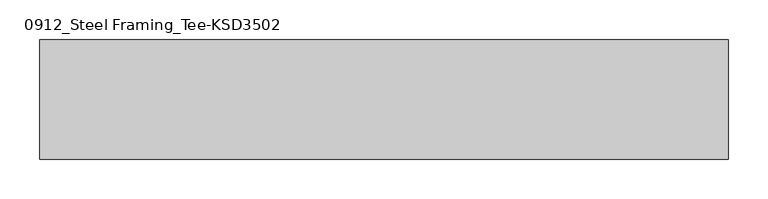
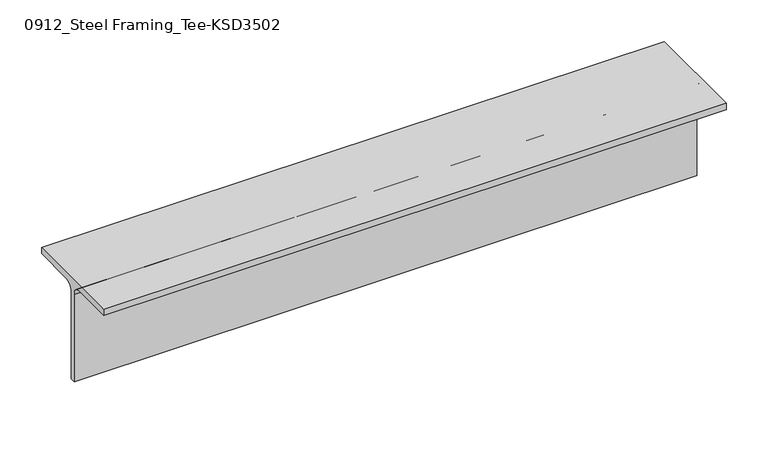
"""IFC4 building model written with IfcOpenShell, lengths in millimetres: member geometry, 0912_Steel Framing_Tee-KSD3502 : H_SB_ASB_CT-150x150x6.5x9."""

from ifc_helpers import new_model, si_unit, point, frame, frame_2d, origin, place, context, project, spatial, polyline, circle_curve, trimmed, segment, composite_curve, outline, extrude, source, transform, mapped, element, save


def member_0912_steel_framing_tee_ksd3502_ed30f98e(model_context):
    return source(origin(), model_context, "Body", "SweptSolid", [
        extrude(outline(composite_curve([segment(polyline([(-75.0, 75.0), (75.0, 75.0), (75.0, 66.0), (16.25, 66.0)]), True, "CONTINUOUS"), segment(trimmed(circle_curve(frame_2d((16.25, 53.0)), 13.0), [point((16.25, 66.0))], [point((3.25, 53.0))], True, "CARTESIAN"), True, "CONTINUOUS"), segment(polyline([(3.25, 53.0), (3.25, -75.0), (-3.25, -75.0), (-3.25, 53.0)]), True, "CONTINUOUS"), segment(trimmed(circle_curve(frame_2d((-16.25, 53.0)), 13.0), [point((-3.25, 53.0))], [point((-16.25, 66.0))], True, "CARTESIAN"), True, "CONTINUOUS"), segment(polyline([(-16.25, 66.0), (-75.0, 66.0), (-75.0, 75.0)]), True, "CONTINUOUS")], self_intersect=False)), frame((-365.9, 0.0, 0.0), z_axis=(1.0, 0.0, 0.0), x_axis=(0.0, 1.0, 0.0)), (0.0, 0.0, 1.0), 865.9),
    ])


if __name__ == "__main__":
    model = new_model("IFC4")
    model_context = context("Model", 3, world=origin())
    ifc_project = project(units=[si_unit("LENGTHUNIT", "METRE", prefix="MILLI")], contexts=[model_context])
    site = spatial("IfcSite", under=ifc_project)
    building = spatial("IfcBuilding", under=site)
    placement = place(None, origin())
    member_0912_steel_framing_tee_ksd3502_shape = member_0912_steel_framing_tee_ksd3502_ed30f98e(model_context)
    element("IfcMember", 1, ObjectType="0912_Steel Framing_Tee-KSD3502 : H_SB_ASB_CT-150x150x6.5x9", at=placement, inside=building, context=model_context, shape_type="MappedRepresentation", body=[
        mapped(member_0912_steel_framing_tee_ksd3502_shape, transform((0.0, 0.0, 0.0), x_axis=(1.0, 0.0, 0.0), y_axis=(0.0, 1.0, 0.0), z_axis=(0.0, 0.0, 1.0))),
    ])
    save(model, "model.ifc")

# Revit data of these elements
# Type "0912_Steel Framing_Tee-KSD3502 : H_SB_ASB_CT-150x150x6.5x9"
#   H_WM Code_1 = "S01AA003-00001 | Main Steel Structure Fabrication Work | Shelter/Building | Light Steel - Standard (30KG/M>Weight) | Material: (   )"
#   H_WM Code_2 = "S03AA029-00001 | Main Steel Structure Erection Work | Shelter/Building | Light Steel (30KG/M>Weight) | Material: (   )"
#   H_WM Code_3 = "S01AA010-00001 | Main Steel Structure Fabrication Work | Shelter/Building | Steel Painting/Coating | for Non-Fireproofed Steel Surface, Surface Preparation, Primer, Second & Final Coat | Material: (   )"
#   H_Q'ty Cal Type Tag = "SB-Q2"
#   Width = 15.0 cm
#   Web Thickness = 0.65 cm
#   Web Fillet = 1.3 cm
#   Section Area = 23.39 cm²
#   Perimeter = 0.60 m²/m
#   Nominal Weight = 18.40 kgf/m
#   Height = 15.0 cm
#   Flange Thickness = 0.9 cm
#   Centroid Vertical = 7.5 cm
#   Centroid Horizontal = 7.5 cm
#   Length [instance default] = 1.5000 m
#   Structural Material [instance default] = Steel, 45-345
#   Warping Constant = (empty or 0)
#   Torsional Moment of Inertia = 0
#   Section Name Key = ""
#   Plastic Modulus weak axis = 0
#   Plastic Modulus strong axis = 0
#   Moment of Inertia weak axis = 0
#   Moment of Inertia strong axis = 0
#   Elastic Modulus weak axis = 0
#   Elastic Modulus strong axis = 0
#   Bolt Spacing = 0
#   Assembly Code = ""
# Element 1 (IfcMember, "0912_Steel Framing_Tee-KSD3502 : H_SB_ASB_CT-150x150x6.5x9")
#   Structural Material = none
# Materials
#   "Steel, 45-345": class "Metal", colour RGB 189 187 185, transparency 0, Description = "Steel 345 MPa", Cost = 0
